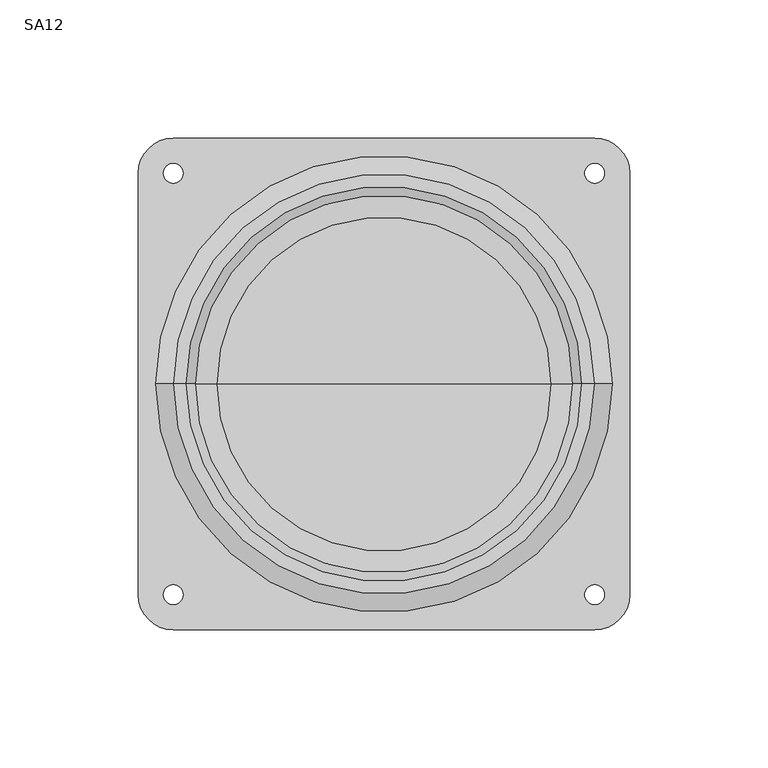
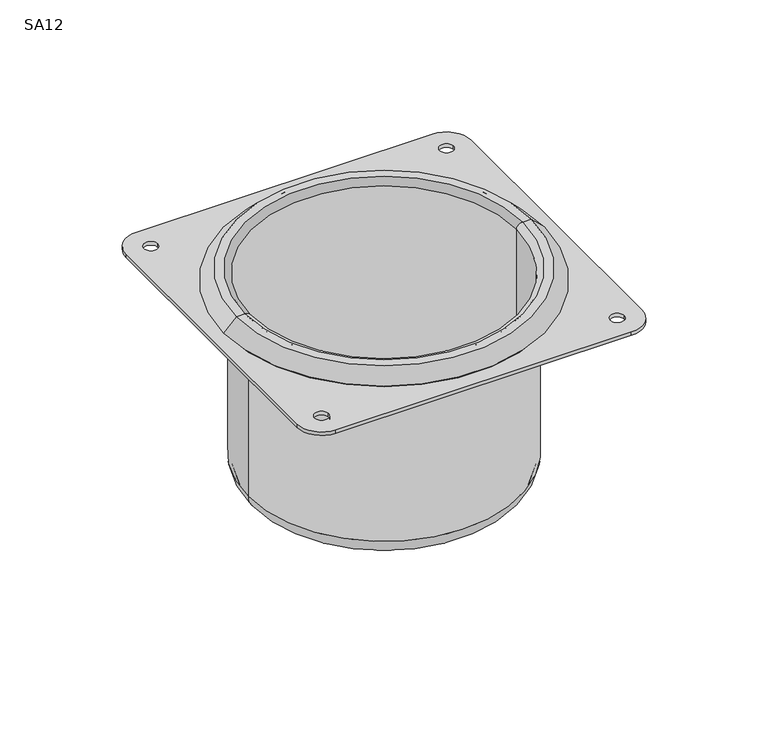
"""IFC4 building model written with IfcOpenShell, lengths in millimetres: proxy geometry, Security_Accessories-Bradley-SA12 : SA12."""

from ifc_helpers import new_model, si_unit, point, frame, frame_2d, origin, origin_with_axes, origin_2d, place, context, project, spatial, polyline, circle_curve, ellipse_curve, trimmed, segment, composite_curve, outline, extrude, source, transform, mapped, element, save
from ifc_brep_helpers import plane_surface, cylinder_surface, revolved_surface, advanced_brep


def sa12_6de3b1ef(model_context):
    return source(origin(), model_context, "Body", "SolidModel", [
        extrude(outline(composite_curve([segment(polyline([(-88.9, -76.2), (-88.9, 76.2)]), True, "CONTINUOUS"), segment(trimmed(circle_curve(frame_2d((-76.2, 76.2)), 12.7), [point((-88.9, 76.2))], [point((-76.2, 88.9))], False, "CARTESIAN"), True, "CONTINUOUS"), segment(polyline([(-76.2, 88.9), (76.2, 88.9)]), True, "CONTINUOUS"), segment(trimmed(circle_curve(frame_2d((76.2, 76.2)), 12.7), [point((76.2, 88.9))], [point((88.9, 76.2))], False, "CARTESIAN"), True, "CONTINUOUS"), segment(polyline([(88.9, 76.2), (88.9, -76.2)]), True, "CONTINUOUS"), segment(trimmed(circle_curve(frame_2d((76.2, -76.2)), 12.7), [point((88.9, -76.2))], [point((76.2, -88.9))], False, "CARTESIAN"), True, "CONTINUOUS"), segment(polyline([(76.2, -88.9), (-76.2, -88.9)]), True, "CONTINUOUS"), segment(trimmed(circle_curve(frame_2d((-76.2, -76.2)), 12.7), [point((-76.2, -88.9))], [point((-88.9, -76.2))], False, "CARTESIAN"), True, "CONTINUOUS")], self_intersect=False), holes=[composite_curve([segment(trimmed(circle_curve(frame_2d((-76.2, -76.2)), 3.571875), [point((-79.771875, -76.2))], [point((-72.628125, -76.2))], True, "CARTESIAN"), True, "CONTINUOUS"), segment(trimmed(circle_curve(frame_2d((-76.2, -76.2)), 3.571875), [point((-72.628125, -76.2))], [point((-79.771875, -76.2))], True, "CARTESIAN"), True, "CONTINUOUS")], self_intersect=False), composite_curve([segment(trimmed(circle_curve(frame_2d((-76.2, 76.2)), 3.571875), [point((-79.771875, 76.2))], [point((-72.628125, 76.2))], True, "CARTESIAN"), True, "CONTINUOUS"), segment(trimmed(circle_curve(frame_2d((-76.2, 76.2)), 3.571875), [point((-72.628125, 76.2))], [point((-79.771875, 76.2))], True, "CARTESIAN"), True, "CONTINUOUS")], self_intersect=False), composite_curve([segment(trimmed(circle_curve(frame_2d((76.2, 76.2)), 3.571875), [point((72.628125, 76.2))], [point((79.771875, 76.2))], True, "CARTESIAN"), True, "CONTINUOUS"), segment(trimmed(circle_curve(frame_2d((76.2, 76.2)), 3.571875), [point((79.771875, 76.2))], [point((72.628125, 76.2))], True, "CARTESIAN"), True, "CONTINUOUS")], self_intersect=False), composite_curve([segment(trimmed(circle_curve(frame_2d((76.2, -76.2)), 3.571875), [point((72.628125, -76.2))], [point((79.771875, -76.2))], True, "CARTESIAN"), True, "CONTINUOUS"), segment(trimmed(circle_curve(frame_2d((76.2, -76.2)), 3.571875), [point((79.771875, -76.2))], [point((72.628125, -76.2))], True, "CARTESIAN"), True, "CONTINUOUS")], self_intersect=False), composite_curve([segment(trimmed(circle_curve(origin_2d(), 81.4723693), [point((-81.4723693, 0.0))], [point((81.4723693, 0.0))], True, "CARTESIAN"), True, "CONTINUOUS"), segment(trimmed(circle_curve(origin_2d(), 81.4723693), [point((81.4723693, 0.0))], [point((-81.4723693, 0.0))], True, "CARTESIAN"), True, "CONTINUOUS")], self_intersect=False)]), origin_with_axes(), (0.0, 0.0, 1.0), 1.905),
        advanced_brep(
        [(68.326, 0.0, 6.4135), (68.326, 0.0, -90.551), (-68.326, 0.0, -90.551), (-68.326, 0.0, 6.4135), (71.4375, 0.0, 9.525), (-71.4375, 0.0, 9.525), (76.0076307, 0.0, 9.525), (-76.0076307, 0.0, 9.525), (82.55, 0.0, 2.9826307), (-82.55, 0.0, 2.9826307), (81.4723693, 0.0, 1.905), (-81.4723693, 0.0, 1.905), (75.3763693, 0.0, 8.001), (-75.3763693, 0.0, 8.001), (71.4375, 0.0, 8.001), (-71.4375, 0.0, 8.001), (69.85, 0.0, 6.4135), (-69.85, 0.0, 6.4135), (69.85, 0.0, -90.551), (-69.85, 0.0, -90.551), (60.3885, 0.0, -100.0125), (-60.3885, 0.0, -100.0125), (0.0, 0.0, -100.0125), (60.3885, 0.0, -98.4885), (0.0, 0.0, -98.4885), (-60.3885, 0.0, -98.4885)],
        [
            (0, 1),
            (1, 2, circle_curve(frame((0.0, 0.0, -90.551), z_axis=(0.0, 0.0, -1.0), x_axis=(-1.0, 0.0, 0.0)), 68.326)),
            (2, 3),
            (3, 0, circle_curve(frame((0.0, 0.0, 6.4135), z_axis=(0.0, 0.0, 1.0), x_axis=(-1.0, 0.0, 0.0)), 68.326)),
            (2, 1, circle_curve(frame((0.0, 0.0, -90.551), z_axis=(0.0, 0.0, -1.0), x_axis=(-1.0, 0.0, 0.0)), 68.326)),
            (0, 3, circle_curve(frame((0.0, 0.0, 6.4135), z_axis=(0.0, 0.0, 1.0), x_axis=(-1.0, 0.0, 0.0)), 68.326)),
            (4, 0, circle_curve(frame((71.4375, 0.0, 6.4135), z_axis=(0.0, -1.0, 0.0), x_axis=(-1.0, 0.0, 0.0)), 3.1115)),
            (3, 5, circle_curve(frame((-71.4375, 0.0, 6.4135), z_axis=(0.0, -1.0, 0.0), x_axis=(1.0, 0.0, 0.0)), 3.1115)),
            (5, 4, circle_curve(frame((0.0, 0.0, 9.525), z_axis=(0.0, 0.0, 1.0), x_axis=(-1.0, 0.0, 0.0)), 71.4375)),
            (4, 5, circle_curve(frame((0.0, 0.0, 9.525), z_axis=(0.0, 0.0, 1.0), x_axis=(-1.0, 0.0, 0.0)), 71.4375)),
            (6, 4),
            (5, 7),
            (7, 6, circle_curve(frame((0.0, 0.0, 9.525), z_axis=(0.0, 0.0, 1.0), x_axis=(-1.0, 0.0, 0.0)), 76.0076307)),
            (6, 7, circle_curve(frame((0.0, 0.0, 9.525), z_axis=(0.0, 0.0, 1.0), x_axis=(-1.0, 0.0, 0.0)), 76.0076307)),
            (8, 6),
            (7, 9),
            (9, 8, circle_curve(frame((0.0, 0.0, 2.9826307), z_axis=(0.0, 0.0, 1.0), x_axis=(-1.0, 0.0, 0.0)), 82.55)),
            (8, 9, circle_curve(frame((0.0, 0.0, 2.9826307), z_axis=(0.0, 0.0, 1.0), x_axis=(-1.0, 0.0, 0.0)), 82.55)),
            (10, 8),
            (9, 11),
            (11, 10, circle_curve(frame((0.0, 0.0, 1.905), z_axis=(0.0, 0.0, 1.0), x_axis=(-1.0, 0.0, 0.0)), 81.4723693)),
            (10, 11, circle_curve(frame((0.0, 0.0, 1.905), z_axis=(0.0, 0.0, 1.0), x_axis=(-1.0, 0.0, 0.0)), 81.4723693)),
            (12, 10),
            (11, 13),
            (13, 12, circle_curve(frame((0.0, 0.0, 8.001), z_axis=(0.0, 0.0, 1.0), x_axis=(-1.0, 0.0, 0.0)), 75.3763693)),
            (12, 13, circle_curve(frame((0.0, 0.0, 8.001), z_axis=(0.0, 0.0, 1.0), x_axis=(-1.0, 0.0, 0.0)), 75.3763693)),
            (14, 12),
            (13, 15),
            (15, 14, circle_curve(frame((0.0, 0.0, 8.001), z_axis=(0.0, 0.0, 1.0), x_axis=(-1.0, 0.0, 0.0)), 71.4375)),
            (14, 15, circle_curve(frame((0.0, 0.0, 8.001), z_axis=(0.0, 0.0, 1.0), x_axis=(-1.0, 0.0, 0.0)), 71.4375)),
            (16, 14, circle_curve(frame((71.4375, 0.0, 6.4135), z_axis=(0.0, 1.0, 0.0), x_axis=(-1.0, 0.0, 0.0)), 1.5875)),
            (15, 17, circle_curve(frame((-71.4375, 0.0, 6.4135), z_axis=(0.0, 1.0, 0.0), x_axis=(1.0, 0.0, 0.0)), 1.5875)),
            (17, 16, circle_curve(frame((0.0, 0.0, 6.4135), z_axis=(0.0, 0.0, 1.0), x_axis=(-1.0, 0.0, 0.0)), 69.85)),
            (16, 17, circle_curve(frame((0.0, 0.0, 6.4135), z_axis=(0.0, 0.0, 1.0), x_axis=(-1.0, 0.0, 0.0)), 69.85)),
            (18, 16),
            (17, 19),
            (19, 18, circle_curve(frame((0.0, 0.0, -90.551), z_axis=(0.0, 0.0, 1.0), x_axis=(-1.0, 0.0, 0.0)), 69.85)),
            (18, 19, circle_curve(frame((0.0, 0.0, -90.551), z_axis=(0.0, 0.0, 1.0), x_axis=(-1.0, 0.0, 0.0)), 69.85)),
            (20, 18, circle_curve(frame((60.3885, 0.0, -90.551), z_axis=(0.0, -1.0, 0.0), x_axis=(-1.0, 0.0, 0.0)), 9.4615)),
            (19, 21, circle_curve(frame((-60.3885, 0.0, -90.551), z_axis=(0.0, -1.0, 0.0), x_axis=(1.0, 0.0, 0.0)), 9.4615)),
            (21, 20, circle_curve(frame((0.0, 0.0, -100.0125), z_axis=(0.0, 0.0, 1.0), x_axis=(-1.0, 0.0, 0.0)), 60.3885)),
            (20, 21, circle_curve(frame((0.0, 0.0, -100.0125), z_axis=(0.0, 0.0, 1.0), x_axis=(-1.0, 0.0, 0.0)), 60.3885)),
            (22, 20),
            (21, 22),
            (23, 24),
            (24, 25),
            (25, 23, circle_curve(frame((0.0, 0.0, -98.4885), z_axis=(0.0, 0.0, 1.0), x_axis=(-1.0, 0.0, 0.0)), 60.3885)),
            (23, 25, circle_curve(frame((0.0, 0.0, -98.4885), z_axis=(0.0, 0.0, 1.0), x_axis=(-1.0, 0.0, 0.0)), 60.3885)),
            (1, 23, circle_curve(frame((60.3885, 0.0, -90.551), z_axis=(0.0, 1.0, 0.0), x_axis=(-1.0, 0.0, 0.0)), 7.9375)),
            (25, 2, circle_curve(frame((-60.3885, 0.0, -90.551), z_axis=(0.0, 1.0, 0.0), x_axis=(1.0, 0.0, 0.0)), 7.9375)),
        ],
        [
            revolved_surface(polyline([(-68.326, 0.0, -90.551), (-68.326, 0.0, 6.413499999999999)]), (0.0, 0.0, -119.0625), (0.0, 0.0, -1.0)),
            revolved_surface(trimmed(ellipse_curve(frame((-71.4375, 0.0, 6.4135), z_axis=(0.0, -1.0, 0.0), x_axis=(1.0, 0.0, 0.0)), 3.1115, 3.1115), [point((-68.326, 0.0, 6.4135))], [point((-71.4375, 0.0, 9.525))], True, "CARTESIAN"), (0.0, 0.0, -119.0625), (0.0, 0.0, -1.0)),
            plane_surface(frame((0.0, 0.0, 9.525), z_axis=(0.0, 0.0, 1.0), x_axis=(-1.0, 0.0, 0.0))),
            revolved_surface(polyline([(-76.0076307, 0.0, 9.525), (-82.55, 0.0, 2.9826307)]), (0.0, 0.0, -119.0625), (0.0, 0.0, -1.0)),
            revolved_surface(polyline([(-82.55, 0.0, 2.9826307), (-81.4723693, 0.0, 1.905)]), (0.0, 0.0, -119.0625), (0.0, 0.0, -1.0)),
            revolved_surface(polyline([(-81.4723693, 0.0, 1.905), (-75.3763693, 0.0, 8.001)]), (0.0, 0.0, -119.0625), (0.0, 0.0, -1.0)),
            plane_surface(frame((0.0, 0.0, 8.001), z_axis=(0.0, 0.0, -1.0), x_axis=(-1.0, 0.0, 0.0))),
            revolved_surface(trimmed(ellipse_curve(frame((-71.4375, 0.0, 6.4135), z_axis=(0.0, 1.0, 0.0), x_axis=(1.0, 0.0, 0.0)), 1.5875, 1.5875), [point((-71.4375, 0.0, 8.001))], [point((-69.85, 0.0, 6.4135))], True, "CARTESIAN"), (0.0, 0.0, -119.0625), (0.0, 0.0, -1.0)),
            cylinder_surface(frame((0.0, 0.0, -119.0625), z_axis=(0.0, 0.0, -1.0), x_axis=(-1.0, 0.0, 0.0)), 69.85),
            revolved_surface(trimmed(ellipse_curve(frame((-60.3885, 0.0, -90.551), z_axis=(0.0, -1.0, 0.0), x_axis=(1.0, 0.0, 0.0)), 9.4615, 9.4615), [point((-69.85, 0.0, -90.551))], [point((-60.3885, 0.0, -100.0125))], True, "CARTESIAN"), (0.0, 0.0, -119.0625), (0.0, 0.0, -1.0)),
            plane_surface(frame((0.0, 0.0, -100.0125), z_axis=(0.0, 0.0, -1.0), x_axis=(-1.0, 0.0, 0.0))),
            plane_surface(frame((0.0, 0.0, -98.4885), z_axis=(0.0, 0.0, 1.0), x_axis=(-1.0, 0.0, 0.0))),
            revolved_surface(trimmed(ellipse_curve(frame((-60.3885, 0.0, -90.551), z_axis=(0.0, 1.0, 0.0), x_axis=(1.0, 0.0, 0.0)), 7.9375, 7.9375), [point((-60.3885, 0.0, -98.4885))], [point((-68.326, 0.0, -90.551))], True, "CARTESIAN"), (0.0, 0.0, -119.0625), (0.0, 0.0, -1.0)),
        ],
        [
            (0, [[1, 2, 3, 4]]),
            (0, [[-3, 5, -1, 6]]),
            (1, [[7, -4, 8, 9]]),
            (1, [[-8, -6, -7, 10]]),
            (2, [[11, -9, 12, 13]]),
            (2, [[-12, -10, -11, 14]]),
            (3, [[15, -13, 16, 17]]),
            (3, [[-16, -14, -15, 18]]),
            (4, [[19, -17, 20, 21]]),
            (4, [[-20, -18, -19, 22]]),
            (5, [[23, -21, 24, 25]]),
            (5, [[-24, -22, -23, 26]]),
            (6, [[27, -25, 28, 29]]),
            (6, [[-28, -26, -27, 30]]),
            (7, [[31, -29, 32, 33]]),
            (7, [[-32, -30, -31, 34]]),
            (8, [[35, -33, 36, 37]]),
            (8, [[-36, -34, -35, 38]]),
            (9, [[39, -37, 40, 41]]),
            (9, [[-40, -38, -39, 42]]),
            (10, [[43, -41, 44]]),
            (10, [[-44, -42, -43]]),
            (11, [[45, 46, 47]]),
            (11, [[-46, -45, 48]]),
            (12, [[49, -47, 50, -2]]),
            (12, [[-50, -48, -49, -5]]),
        ],
    ),
    ])


if __name__ == "__main__":
    model = new_model("IFC4")
    model_context = context("Model", 3, world=origin())
    ifc_project = project(units=[si_unit("LENGTHUNIT", "METRE", prefix="MILLI")], contexts=[model_context])
    site = spatial("IfcSite", under=ifc_project)
    building = spatial("IfcBuilding", under=site)
    placement = place(None, origin())
    sa12_shape = sa12_6de3b1ef(model_context)
    element("IfcBuildingElementProxy", 1, Name="Security_Accessories-Bradley-SA12 : SA12", ObjectType="Security_Accessories-Bradley-SA12 : SA12", at=placement, inside=building, context=model_context, shape_type="MappedRepresentation", body=[
        mapped(sa12_shape, transform((0.0, 0.0, 0.0), x_axis=(1.0, 0.0, 0.0), y_axis=(0.0, 1.0, 0.0), z_axis=(0.0, 0.0, 1.0))),
    ])
    save(model, "model.ifc")

# Revit data of these elements
# Type "Security_Accessories-Bradley-SA12 : SA12"
#   Warranty Information = "Complete Unit - One Year"
#   Version = "1.0"
#   URL = "http://www.bradleycorp.com/"
#   OmniClass Title = "Toilet Tissue Dispensers"
#   OmniClass Code = "23.21.43.15.31"
#   Modeling Code = ""
#   Model = "SA12"
#   MasterFormat Title = "Security Toilet Accessories"
#   MasterFormat Number = "10 28 13.53"
#   Manufacturer = "Bradley Corporation"
#   Industry Standards = ""
#   Fire Rating = ""
#   Description = "Security Toilet Tissue Roll Holder"
#   Copyright = "This Model Data is Property of Bradley Corporation"
#   Buy American Act = "Yes"
#   Assembly Code = "C1030200"
#   ADA Compliant = "Yes"
#   Width = 177.8 mm
#   Height = 177.8 mm
#   Default Elevation = 1219.2 mm
#   Material = Metal - Bradley Corp - Stainless Steel - Satin
# Element 1 (IfcBuildingElementProxy, "Security_Accessories-Bradley-SA12 : SA12")
#   Materials on its faces: "Metal - Bradley Corp - Stainless Steel - Satin"
# Materials
#   "Metal - Bradley Corp - Stainless Steel - Satin": class "Metal", colour RGB 189 187 185, transparency 0, Manufacturer = "Bradley Corporation", URL = "www.bradleycorp.com", Description = "Stainless Steel - Satin Finish", Cost = 0
